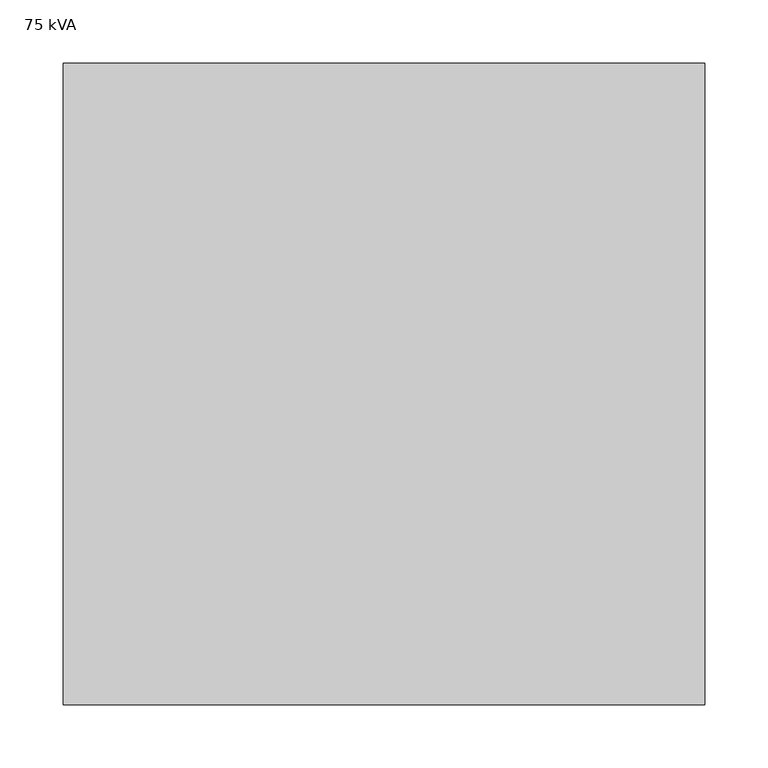
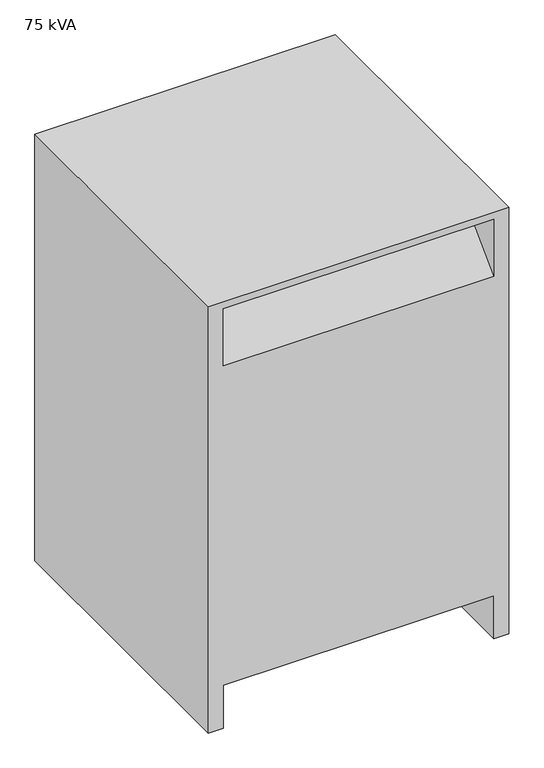
"""IFC4 building model written with IfcOpenShell, lengths in millimetres: proxy geometry, Dry Type Transformer - 480-208Y120 - NEMA Type 2 : 75 kVA."""

from ifc_helpers import new_model, si_unit, origin, place, context, project, spatial, faceted_brep, source, transform, mapped, element, save


def proxy_75_kva_f23e4866(model_context):
    return source(origin(), model_context, "Body", "Brep", [
        faceted_brep([(254.0, -123.2841349, 762.0), (254.0, 384.7158651, 762.0), (-254.0, 384.7158651, 762.0), (-254.0, -123.2841349, 762.0), (-254.0, -123.2841349, 0.0), (-254.0, 384.7158651, 0.0), (-228.6, 384.7158651, 0.0), (-228.6, -123.2841349, 0.0), (254.0, 384.7158651, 0.0), (254.0, -123.2841349, 0.0), (228.6, -123.2841349, 0.0), (228.6, 384.7158651, 0.0), (228.6, 384.7158651, 76.2), (-228.6, 384.7158651, 76.2), (228.6, 384.7158651, 647.7), (228.6, 384.7158651, 749.3), (-228.6, 384.7158651, 749.3), (-228.6, 384.7158651, 647.7), (-228.6, -123.2841349, 76.2), (228.6, -123.2841349, 76.2), (228.6, -123.2841349, 749.3), (228.6, -123.2841349, 647.7), (-228.6, -123.2841349, 647.7), (-228.6, -123.2841349, 749.3), (228.6, -21.6841349, 749.3), (-228.6, -21.6841349, 749.3), (228.6, 283.1158651, 749.3), (-228.6, 283.1158651, 749.3)], [[[0, 1, 2, 3]], [[4, 5, 6, 7]], [[8, 9, 10, 11]], [[1, 0, 9, 8]], [[2, 1, 8, 11, 12, 13, 6, 5], [14, 15, 16, 17]], [[3, 2, 5, 4]], [[0, 3, 4, 7, 18, 19, 10, 9], [20, 21, 22, 23]], [[18, 13, 12, 19]], [[13, 18, 7, 6]], [[19, 12, 11, 10]], [[24, 21, 20]], [[25, 23, 22]], [[24, 20, 23, 25]], [[21, 24, 25, 22]], [[26, 15, 14]], [[27, 17, 16]], [[26, 14, 17, 27]], [[15, 26, 27, 16]]]),
    ])


if __name__ == "__main__":
    model = new_model("IFC4")
    model_context = context("Model", 3, world=origin())
    ifc_project = project(units=[si_unit("LENGTHUNIT", "METRE", prefix="MILLI")], contexts=[model_context])
    site = spatial("IfcSite", under=ifc_project)
    building = spatial("IfcBuilding", under=site)
    placement = place(None, origin())
    proxy_75_kva_shape = proxy_75_kva_f23e4866(model_context)
    element("IfcBuildingElementProxy", 1, Name="Dry Type Transformer - 480-208Y120 - NEMA Type 2 : 75 kVA", ObjectType="Dry Type Transformer - 480-208Y120 - NEMA Type 2 : 75 kVA", at=placement, inside=building, context=model_context, shape_type="MappedRepresentation", body=[
        mapped(proxy_75_kva_shape, transform((0.0, 0.0, 0.0), x_axis=(1.0, 0.0, 0.0), y_axis=(0.0, 1.0, 0.0), z_axis=(0.0, 0.0, 1.0))),
    ])
    save(model, "model.ifc")

# Revit data of these elements
# Project information
#   Project Issue Date = "Issue Date"
#   Project Status = "Project Status"
#   Client Name = "Owner"
#   Project Address = "Enter address here"
#   Project Name = "Project Name"
#   Project Number = "Project Number"
# Type "Dry Type Transformer - 480-208Y120 - NEMA Type 2 : 75 kVA"
#   built-in parameter 1140083 [instance default] = "Type 2"
#   Transformer Length = 1' - 8"
#   Primary Voltage = 480 V
#   Transformer Height = 2' - 6"
#   built-in parameter 1140140 [instance default] = 1 (stored number, unit not read)
#   Transformer Width = 1' - 8"
#   built-in parameter 1140142 [instance default] = -1
#   Primary Number of Poles = 3
#   built-in parameter 1140079 [instance default] = 3
#   Transformer Material = none
#   Load Classification = Transformer
#   Default Elevation = 0
#   Assembly Code = ""
#   built-in parameter 1140087 [instance default] = 1
